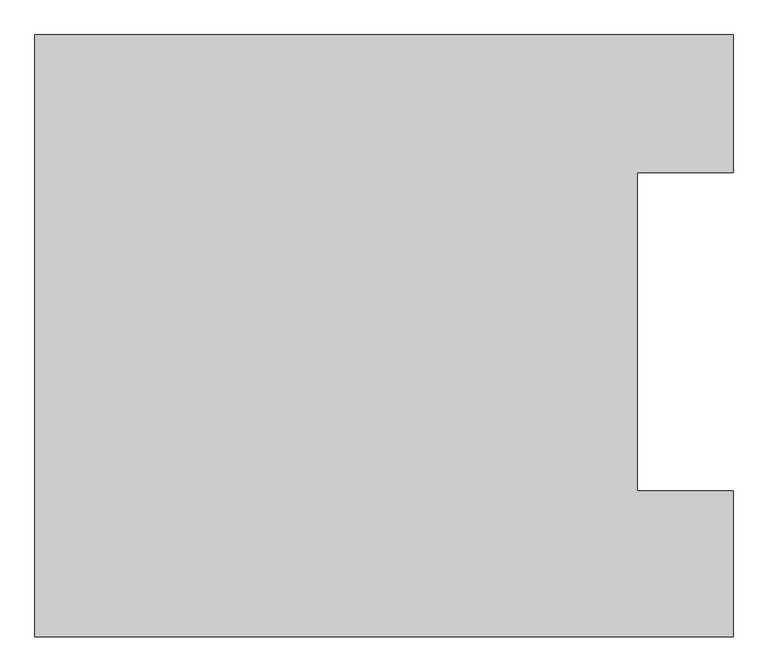
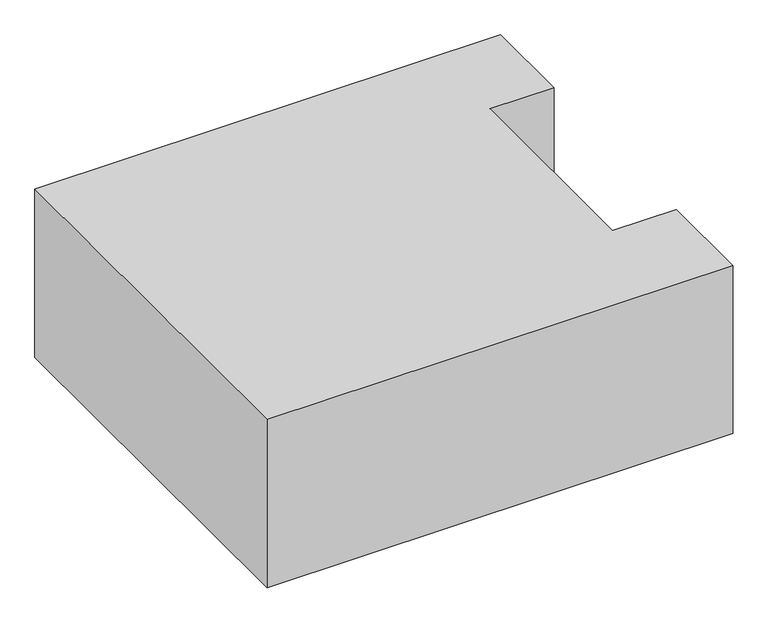
"""IFC4 building model written with IfcOpenShell, lengths in millimetres: proxy geometry, 0_3d_modell."""

import ifcopenshell
import ifcopenshell.guid

model = None  # the IFC model being written
_history = None  # IfcOwnerHistory: only IFC2X3 demands one
_inside = {}  # id of a spatial element -> (the spatial element, [elements in it])
_under = {}  # id of a project, library or spatial element -> (it, [spatial elements below it])
_declared = {}  # id of a project -> (the project, [libraries it declares])
_typed = {}  # id of a type object -> (the type object, [elements of that type])
_made_of = {}  # id of a material, layer set ... -> (it, [elements and type objects made of it])


def new_model(schema):
    """Start an empty IFC model of exactly this schema.

    Asked for "IFC4X3", IfcOpenShell would pick the latest addendum, in which some entities
    have other attributes; the version numbers below select the first issue.
    IFC2X3 requires an IfcOwnerHistory on every rooted entity: one is made here for all.
    """
    global model, _history
    if schema == "IFC4X3":
        model = ifcopenshell.file(schema_version=(4, 3, 0, 0))
    else:
        model = ifcopenshell.file(schema=schema)
    _inside.clear()
    _under.clear()
    _declared.clear()
    _typed.clear()
    _made_of.clear()
    _history = None
    if model.schema == "IFC2X3":
        org = make("IfcOrganization", Name="unknown")
        user = make(
            "IfcPersonAndOrganization",
            ThePerson=make("IfcPerson", FamilyName="unknown"),
            TheOrganization=org,
        )
        app = make(
            "IfcApplication",
            ApplicationDeveloper=org,
            Version="unknown",
            ApplicationFullName="unknown",
            ApplicationIdentifier="unknown",
        )
        _history = make(
            "IfcOwnerHistory",
            OwningUser=user,
            OwningApplication=app,
            ChangeAction="ADDED",
            CreationDate=0,
        )
    return model


def make(cls, **values):
    """One entity of the class cls with the attributes given. An attribute that is None is left unset."""
    return model.create_entity(
        cls, **{name: value for name, value in values.items() if value is not None}
    )


def rooted(cls, **values):
    """An entity with a GlobalId (a new one), such as an element, a storey or a relation."""
    return make(cls, GlobalId=ifcopenshell.guid.new(), OwnerHistory=_history, **values)


def si_unit(unit_type, name, prefix=None):
    """IfcSIUnit, for example si_unit("LENGTHUNIT", "METRE", prefix="MILLI")."""
    return make("IfcSIUnit", UnitType=unit_type, Prefix=prefix, Name=name)


def assignment(units):
    """IfcUnitAssignment: the units of a project."""
    return None if units is None else make("IfcUnitAssignment", Units=units)


def point(xyz):
    """IfcCartesianPoint."""
    return None if xyz is None else make("IfcCartesianPoint", Coordinates=xyz)


def direction(xyz):
    """IfcDirection."""
    return None if xyz is None else make("IfcDirection", DirectionRatios=xyz)


def frame(location, z_axis=None, x_axis=None):
    """IfcAxis2Placement3D, a coordinate frame: its origin and axes. An axis left out is left unset."""
    return make(
        "IfcAxis2Placement3D",
        Location=point(location),
        Axis=direction(z_axis),
        RefDirection=direction(x_axis),
    )


def origin():
    """The frame at (0, 0, 0) with its axes left unset."""
    return frame((0.0, 0.0, 0.0))


def origin_with_axes():
    """The frame at (0, 0, 0) with the z axis (0, 0, 1) and the x axis (1, 0, 0) written out."""
    return frame((0.0, 0.0, 0.0), z_axis=(0.0, 0.0, 1.0), x_axis=(1.0, 0.0, 0.0))


def place(relative_to, where):
    """IfcLocalPlacement: puts the frame where relative to a parent placement (None: the world)."""
    return make(
        "IfcLocalPlacement", PlacementRelTo=relative_to, RelativePlacement=where
    )


def context(
    kind, dimensions, precision=None, world=None, true_north=None, identifier=None
):
    """IfcGeometricRepresentationContext, for example the 3D "Model" context."""
    return make(
        "IfcGeometricRepresentationContext",
        ContextIdentifier=identifier,
        ContextType=kind,
        CoordinateSpaceDimension=dimensions,
        Precision=precision,
        WorldCoordinateSystem=world,
        TrueNorth=true_north,
    )


def project(units=None, contexts=None):
    """IfcProject with its units and contexts."""
    return rooted(
        "IfcProject",
        Name="project",
        RepresentationContexts=contexts,
        UnitsInContext=assignment(units),
    )


def spatial(cls, under=None, at=None, **own):
    """A site, building, storey or space (cls), placed at a placement, below another one or the project."""
    s = rooted(cls, ObjectPlacement=at, **own)
    if under is not None:
        _under.setdefault(under.id(), (under, []))[1].append(s)
    return s


def polyline(points):
    """IfcPolyline through the points."""
    return make("IfcPolyline", Points=[point(p) for p in points])


def outline(outer, holes=None, kind="AREA"):
    """IfcArbitraryClosedProfileDef: a profile drawn as a closed curve; with holes, ...WithVoids."""
    if holes is None:
        return make("IfcArbitraryClosedProfileDef", ProfileType=kind, OuterCurve=outer)
    return make(
        "IfcArbitraryProfileDefWithVoids",
        ProfileType=kind,
        OuterCurve=outer,
        InnerCurves=holes,
    )


def extrude(swept, where, along, depth):
    """IfcExtrudedAreaSolid: the profile swept, set in the frame where, extruded along a direction by depth."""
    return make(
        "IfcExtrudedAreaSolid",
        SweptArea=swept,
        Position=where,
        ExtrudedDirection=direction(along),
        Depth=depth,
    )


def shape(context_of_items, identifier, shape_type, items):
    """IfcShapeRepresentation: the items that make up one representation, for example the "Body"."""
    return make(
        "IfcShapeRepresentation",
        ContextOfItems=context_of_items,
        RepresentationIdentifier=identifier,
        RepresentationType=shape_type,
        Items=items,
    )


def source(mapping_origin, context_of_items, identifier, shape_type, items):
    """IfcRepresentationMap: a shape defined once, which mapped items show again and again."""
    return make(
        "IfcRepresentationMap",
        MappingOrigin=mapping_origin,
        MappedRepresentation=shape(context_of_items, identifier, shape_type, items),
    )


def transform(
    local_origin,
    x_axis=None,
    y_axis=None,
    z_axis=None,
    scale=None,
    scale2=None,
    scale3=None,
    uniform=True,
):
    """IfcCartesianTransformationOperator3D, or its non-uniform kind. x_axis, y_axis, z_axis: its Axis1, 2, 3."""
    if uniform:
        return make(
            "IfcCartesianTransformationOperator3D",
            Axis1=direction(x_axis),
            Axis2=direction(y_axis),
            LocalOrigin=point(local_origin),
            Scale=scale,
            Axis3=direction(z_axis),
        )
    return make(
        "IfcCartesianTransformationOperator3DnonUniform",
        Axis1=direction(x_axis),
        Axis2=direction(y_axis),
        LocalOrigin=point(local_origin),
        Scale=scale,
        Axis3=direction(z_axis),
        Scale2=scale2,
        Scale3=scale3,
    )


def mapped(mapping_source, mapping_target):
    """IfcMappedItem: shows the shape of a source again, moved by a transform."""
    return make(
        "IfcMappedItem", MappingSource=mapping_source, MappingTarget=mapping_target
    )


def made_of(thing, what):
    """Note that an element or type object is made of a material, layer set ...; save() writes the relation."""
    if what is not None:
        _made_of.setdefault(what.id(), (what, []))[1].append(thing)
    return thing


def element(
    cls,
    number,
    at=None,
    inside=None,
    cuts=None,
    type_object=None,
    material=None,
    context=None,
    identifier="Body",
    shape_type=None,
    held_by="IfcProductDefinitionShape",
    body=None,
    shapes=None,
    **own,
):
    """One element of the class cls, such as IfcWall. Its Tag is "e" and its number.

    at: its placement. inside: the storey or other place that contains it. cuts: it is an
    opening in that element (IfcRelVoidsElement). A single representation is given by context,
    identifier, shape_type and body (its items); several are given by shapes. held_by: the class
    of the entity that holds the representations. save() writes the other relations.
    """
    e = rooted(cls, Tag="e%d" % number, ObjectPlacement=at, **own)
    if body is not None:
        shapes = [shape(context, identifier, shape_type, body)]
    if shapes is not None:
        e.Representation = make(held_by, Representations=shapes)
    if inside is not None:
        _inside.setdefault(inside.id(), (inside, []))[1].append(e)
    if cuts is not None:
        rooted(
            "IfcRelVoidsElement", RelatingBuildingElement=cuts, RelatedOpeningElement=e
        )
    if type_object is not None:
        _typed.setdefault(type_object.id(), (type_object, []))[1].append(e)
    return made_of(e, material)


def aggregate(whole, parts):
    """IfcRelAggregates: a whole, such as a stair, and the parts it consists of."""
    return rooted("IfcRelAggregates", RelatingObject=whole, RelatedObjects=parts)


def save(model, path):
    """Write the relations noted so far, then the file.

    IfcRelAggregates (storeys below a building ...), IfcRelContainedInSpatialStructure (elements
    in a storey), IfcRelDefinesByType, IfcRelAssociatesMaterial and IfcRelDeclares: one each for
    every whole, place, type object, material and project.
    """
    for whole, parts in _under.values():
        aggregate(whole, parts)
    for where, things in _inside.values():
        rooted(
            "IfcRelContainedInSpatialStructure",
            RelatedElements=things,
            RelatingStructure=where,
        )
    for kind, things in _typed.values():
        rooted("IfcRelDefinesByType", RelatedObjects=things, RelatingType=kind)
    for what, things in _made_of.values():
        rooted("IfcRelAssociatesMaterial", RelatedObjects=things, RelatingMaterial=what)
    for by, libraries in _declared.values():
        rooted("IfcRelDeclares", RelatingContext=by, RelatedDefinitions=libraries)
    model.write(path)


def generic_models_2dafeef2(model_context):
    return source(origin(), model_context, "Body", "SweptSolid", [
        extrude(outline(polyline([(6550.0, 0.0), (0.0, 0.0), (0.0, 5650.0), (6550.0, 5650.0), (6550.0, 4357.8), (5650.0, 4357.8), (5650.0, 1367.8), (6550.0, 1367.8), (6550.0, 0.0)])), origin_with_axes(), (0.0, 0.0, 1.0), 2500.0),
    ])


if __name__ == "__main__":
    model = new_model("IFC4")
    model_context = context("Model", 3, world=origin())
    ifc_project = project(units=[si_unit("LENGTHUNIT", "METRE", prefix="MILLI")], contexts=[model_context])
    site = spatial("IfcSite", under=ifc_project)
    building = spatial("IfcBuilding", under=site)
    placement = place(None, origin())
    generic_models_shape = generic_models_2dafeef2(model_context)
    element("IfcBuildingElementProxy", 1, Name="0_3d_modell", ObjectType="0_3d_modell", at=placement, inside=building, context=model_context, shape_type="MappedRepresentation", body=[
        mapped(generic_models_shape, transform((0.0, 0.0, 0.0), x_axis=(1.0, 0.0, 0.0), y_axis=(0.0, 1.0, 0.0), z_axis=(0.0, 0.0, 1.0))),
    ])
    save(model, "model.ifc")

# Revit data of these elements
# Element 1 (IfcBuildingElementProxy, "0_3d_modell")
#   Materials on its faces: "*1"
# Materials
#   "*1": class "Unassigned", colour RGB 175 175 175, transparency 0
